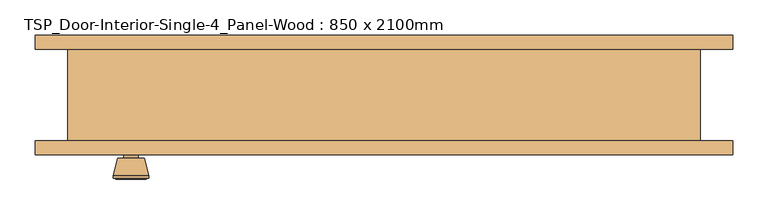
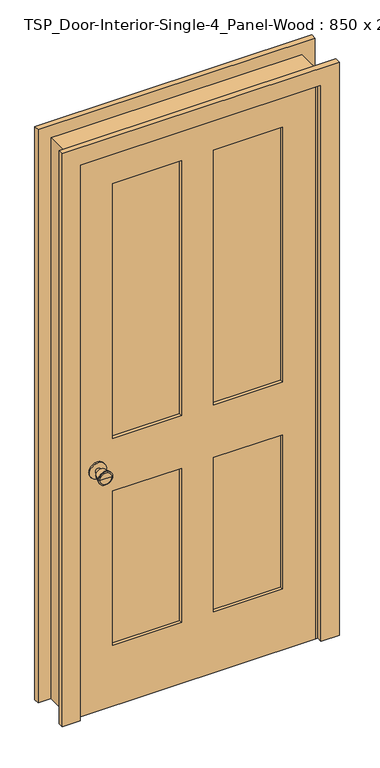
"""IFC4 building model written with IfcOpenShell, lengths in millimetres: door geometry, TSP_Door-Interior-Single-4_Panel-Wood : 850 x 2100mm."""

from ifc_helpers import new_model, si_unit, point, frame, frame_2d, origin, place, context, project, spatial, polyline, circle_curve, trimmed, segment, composite_curve, outline, extrude, faceted_brep, source, transform, mapped, element, save
from ifc_brep_helpers import plane_surface, cylinder_surface, revolved_surface, advanced_brep


def tsp_door_interior_single_4_panel_wood_850_x_2100mm_3b2ec1ce(model_context):
    return source(origin(), model_context, "Body", "SolidModel", [
        advanced_brep(
        [(-360.0, -20.825, 914.4), (-370.0, -20.825, 914.4), (-350.0, -20.825, 914.4), (-339.5241324, 28.175, 914.4), (-380.4758676, 28.175, 914.4), (-360.0, 28.175, 914.4), (-335.0, 26.3471319, 914.4), (-385.0, 26.3471319, 914.4), (-335.0, 22.8834537, 914.4), (-385.0, 22.8834537, 914.4), (-341.363764, -1.825, 914.4), (-378.636236, -1.825, 914.4), (-350.0, -1.825, 914.4), (-370.0, -1.825, 914.4)],
        [
            (0, 1),
            (1, 2, circle_curve(frame((-360.0, -20.825, 914.4), z_axis=(0.0, -1.0, 0.0), x_axis=(-1.0, 0.0, 0.0)), 10.0)),
            (2, 0),
            (2, 1, circle_curve(frame((-360.0, -20.825, 914.4), z_axis=(0.0, -1.0, 0.0), x_axis=(-1.0, 0.0, 0.0)), 10.0)),
            (3, 4, circle_curve(frame((-360.0, 28.175, 914.4), z_axis=(0.0, 1.0, 0.0), x_axis=(-1.0, 0.0, 0.0)), 20.4758676)),
            (4, 5),
            (5, 3),
            (4, 3, circle_curve(frame((-360.0, 28.175, 914.4), z_axis=(0.0, 1.0, 0.0), x_axis=(-1.0, 0.0, 0.0)), 20.4758676)),
            (6, 7, circle_curve(frame((-360.0, 26.3471319, 914.4), z_axis=(0.0, 1.0, 0.0), x_axis=(-1.0, 0.0, 0.0)), 25.0)),
            (7, 4),
            (3, 6),
            (7, 6, circle_curve(frame((-360.0, 26.3471319, 914.4), z_axis=(0.0, 1.0, 0.0), x_axis=(-1.0, 0.0, 0.0)), 25.0)),
            (8, 9, circle_curve(frame((-360.0, 22.8834537, 914.4), z_axis=(0.0, 1.0, 0.0), x_axis=(-1.0, 0.0, 0.0)), 25.0)),
            (9, 7),
            (6, 8),
            (9, 8, circle_curve(frame((-360.0, 22.8834537, 914.4), z_axis=(0.0, 1.0, 0.0), x_axis=(-1.0, 0.0, 0.0)), 25.0)),
            (10, 11, circle_curve(frame((-360.0, -1.825, 914.4), z_axis=(0.0, 1.0, 0.0), x_axis=(-1.0, 0.0, 0.0)), 18.636236)),
            (11, 9),
            (8, 10),
            (11, 10, circle_curve(frame((-360.0, -1.825, 914.4), z_axis=(0.0, 1.0, 0.0), x_axis=(-1.0, 0.0, 0.0)), 18.636236)),
            (12, 13, circle_curve(frame((-360.0, -1.825, 914.4), z_axis=(0.0, 1.0, 0.0), x_axis=(-1.0, 0.0, 0.0)), 10.0)),
            (13, 11),
            (10, 12),
            (13, 12, circle_curve(frame((-360.0, -1.825, 914.4), z_axis=(0.0, 1.0, 0.0), x_axis=(-1.0, 0.0, 0.0)), 10.0)),
            (1, 13),
            (12, 2),
        ],
        [
            plane_surface(frame((-360.0, -20.825, 914.4), z_axis=(0.0, -1.0, 0.0), x_axis=(-1.0, 0.0, 0.0))),
            plane_surface(frame((-360.0, 28.175, 914.4), z_axis=(0.0, 1.0, 0.0), x_axis=(-1.0, 0.0, 0.0))),
            revolved_surface(polyline([(-380.4758676, 28.175, 914.4), (-385.0, 26.3471319, 914.4)]), (-360.0, -20.825, 914.4), (0.0, -1.0, 0.0)),
            cylinder_surface(frame((-360.0, -20.825, 914.4), z_axis=(0.0, -1.0, 0.0), x_axis=(-1.0, 0.0, 0.0)), 25.0),
            revolved_surface(polyline([(-385.0, 22.8834537, 914.4), (-378.636236, -1.825, 914.4)]), (-360.0, -20.825, 914.4), (0.0, -1.0, 0.0)),
            plane_surface(frame((-360.0, -1.825, 914.4), z_axis=(0.0, -1.0, 0.0), x_axis=(-1.0, 0.0, 0.0))),
            cylinder_surface(frame((-360.0, -20.825, 914.4), z_axis=(0.0, -1.0, 0.0), x_axis=(-1.0, 0.0, 0.0)), 10.0),
        ],
        [
            (0, [[1, 2, 3]]),
            (0, [[-3, 4, -1]]),
            (1, [[5, 6, 7]]),
            (1, [[8, -7, -6]]),
            (2, [[9, 10, -5, 11]]),
            (2, [[12, -11, -8, -10]]),
            (3, [[13, 14, -9, 15]]),
            (3, [[16, -15, -12, -14]]),
            (4, [[17, 18, -13, 19]]),
            (4, [[20, -19, -16, -18]]),
            (5, [[21, 22, -17, 23]]),
            (5, [[24, -23, -20, -22]]),
            (6, [[-2, 25, -21, 26]]),
            (6, [[-4, -26, -24, -25]]),
        ],
    ),
        extrude(outline(composite_curve([segment(trimmed(circle_curve(frame_2d((914.4, -360.0)), 30.0), [point((914.4, -390.0))], [point((914.4, -330.0))], False, "CARTESIAN"), True, "CONTINUOUS"), segment(trimmed(circle_curve(frame_2d((914.4, -360.0)), 30.0), [point((914.4, -330.0))], [point((914.4, -390.0))], False, "CARTESIAN"), True, "CONTINUOUS")], self_intersect=False)), frame((0.0, -26.825, 0.0), z_axis=(0.0, 1.0, 0.0), x_axis=(0.0, 0.0, 1.0)), (0.0, 0.0, 1.0), 6.0),
        advanced_brep(
        [(-360.0, -67.825, 914.4), (-350.0, -67.825, 914.4), (-370.0, -67.825, 914.4), (-339.5241324, -116.825, 914.4), (-360.0, -116.825, 914.4), (-380.4758676, -116.825, 914.4), (-335.0, -114.9971319, 914.4), (-385.0, -114.9971319, 914.4), (-335.0, -111.5334537, 914.4), (-385.0, -111.5334537, 914.4), (-341.363764, -86.825, 914.4), (-378.636236, -86.825, 914.4), (-350.0, -86.825, 914.4), (-370.0, -86.825, 914.4)],
        [
            (0, 1),
            (1, 2, circle_curve(frame((-360.0, -67.825, 914.4), z_axis=(0.0, 1.0, 0.0), x_axis=(-1.0, 0.0, 0.0)), 10.0)),
            (2, 0),
            (2, 1, circle_curve(frame((-360.0, -67.825, 914.4), z_axis=(0.0, 1.0, 0.0), x_axis=(-1.0, 0.0, 0.0)), 10.0)),
            (3, 4),
            (4, 5),
            (5, 3, circle_curve(frame((-360.0, -116.825, 914.4), z_axis=(0.0, -1.0, 0.0), x_axis=(-1.0, 0.0, 0.0)), 20.4758676)),
            (3, 5, circle_curve(frame((-360.0, -116.825, 914.4), z_axis=(0.0, -1.0, 0.0), x_axis=(-1.0, 0.0, 0.0)), 20.4758676)),
            (6, 3),
            (5, 7),
            (7, 6, circle_curve(frame((-360.0, -114.9971319, 914.4), z_axis=(0.0, -1.0, 0.0), x_axis=(-1.0, 0.0, 0.0)), 25.0)),
            (6, 7, circle_curve(frame((-360.0, -114.9971319, 914.4), z_axis=(0.0, -1.0, 0.0), x_axis=(-1.0, 0.0, 0.0)), 25.0)),
            (8, 6),
            (7, 9),
            (9, 8, circle_curve(frame((-360.0, -111.5334537, 914.4), z_axis=(0.0, -1.0, 0.0), x_axis=(-1.0, 0.0, 0.0)), 25.0)),
            (8, 9, circle_curve(frame((-360.0, -111.5334537, 914.4), z_axis=(0.0, -1.0, 0.0), x_axis=(-1.0, 0.0, 0.0)), 25.0)),
            (10, 8),
            (9, 11),
            (11, 10, circle_curve(frame((-360.0, -86.825, 914.4), z_axis=(0.0, -1.0, 0.0), x_axis=(-1.0, 0.0, 0.0)), 18.636236)),
            (10, 11, circle_curve(frame((-360.0, -86.825, 914.4), z_axis=(0.0, -1.0, 0.0), x_axis=(-1.0, 0.0, 0.0)), 18.636236)),
            (12, 10),
            (11, 13),
            (13, 12, circle_curve(frame((-360.0, -86.825, 914.4), z_axis=(0.0, -1.0, 0.0), x_axis=(-1.0, 0.0, 0.0)), 10.0)),
            (12, 13, circle_curve(frame((-360.0, -86.825, 914.4), z_axis=(0.0, -1.0, 0.0), x_axis=(-1.0, 0.0, 0.0)), 10.0)),
            (1, 12),
            (13, 2),
        ],
        [
            plane_surface(frame((-360.0, -67.825, 914.4), z_axis=(0.0, 1.0, 0.0), x_axis=(-1.0, 0.0, 0.0))),
            plane_surface(frame((-360.0, -116.825, 914.4), z_axis=(0.0, -1.0, 0.0), x_axis=(-1.0, 0.0, 0.0))),
            revolved_surface(polyline([(-380.4758676, -116.825, 914.4), (-385.0, -114.9971319, 914.4)]), (-360.0, -67.825, 914.4), (0.0, 1.0, 0.0)),
            cylinder_surface(frame((-360.0, -67.825, 914.4), z_axis=(0.0, 1.0, 0.0), x_axis=(-1.0, 0.0, 0.0)), 25.0),
            revolved_surface(polyline([(-385.0, -111.5334537, 914.4), (-378.636236, -86.825, 914.4)]), (-360.0, -67.825, 914.4), (0.0, 1.0, 0.0)),
            plane_surface(frame((-360.0, -86.825, 914.4), z_axis=(0.0, 1.0, 0.0), x_axis=(-1.0, 0.0, 0.0))),
            cylinder_surface(frame((-360.0, -67.825, 914.4), z_axis=(0.0, 1.0, 0.0), x_axis=(-1.0, 0.0, 0.0)), 10.0),
        ],
        [
            (0, [[1, 2, 3]]),
            (0, [[-3, 4, -1]]),
            (1, [[5, 6, 7]]),
            (1, [[-6, -5, 8]]),
            (2, [[9, -7, 10, 11]]),
            (2, [[-10, -8, -9, 12]]),
            (3, [[13, -11, 14, 15]]),
            (3, [[-14, -12, -13, 16]]),
            (4, [[17, -15, 18, 19]]),
            (4, [[-18, -16, -17, 20]]),
            (5, [[21, -19, 22, 23]]),
            (5, [[-22, -20, -21, 24]]),
            (6, [[25, -23, 26, -2]]),
            (6, [[-26, -24, -25, -4]]),
        ],
    ),
        extrude(outline(composite_curve([segment(trimmed(circle_curve(frame_2d((914.4, -360.0)), 30.0), [point((914.4, -390.0))], [point((914.4, -330.0))], False, "CARTESIAN"), True, "CONTINUOUS"), segment(trimmed(circle_curve(frame_2d((914.4, -360.0)), 30.0), [point((914.4, -330.0))], [point((914.4, -390.0))], False, "CARTESIAN"), True, "CONTINUOUS")], self_intersect=False)), frame((0.0, -67.825, 0.0), z_axis=(0.0, 1.0, 0.0), x_axis=(0.0, 0.0, 1.0)), (0.0, 0.0, 1.0), 6.0),
        faceted_brep([(450.0, -61.825, 0.0), (425.0, -61.825, 0.0), (425.0, -26.825, 0.0), (412.3, -26.825, 0.0), (412.3, 8.1, 0.0), (425.0, 8.1, 0.0), (425.0, 68.175, 0.0), (450.0, 68.175, 0.0), (450.0, 68.175, 2125.0), (450.0, -61.825, 2125.0), (425.0, 68.175, 2100.0), (-425.0, 68.175, 2100.0), (-425.0, 68.175, 0.0), (-450.0, 68.175, 0.0), (-450.0, 68.175, 2125.0), (425.0, 8.1, 2100.0), (412.3, 8.1, 2087.3), (-412.3, 8.1, 2087.3), (-412.3, 8.1, 0.0), (-425.0, 8.1, 0.0), (-425.0, 8.1, 2100.0), (412.3, -26.825, 2087.3), (425.0, -26.825, 2100.0), (-425.0, -26.825, 2100.0), (-425.0, -26.825, 0.0), (-412.3, -26.825, 0.0), (-412.3, -26.825, 2087.3), (425.0, -61.825, 2100.0), (-450.0, -61.825, 2125.0), (-450.0, -61.825, 0.0), (-425.0, -61.825, 0.0), (-425.0, -61.825, 2100.0)], [[[0, 1, 2, 3, 4, 5, 6, 7]], [[7, 8, 9, 0]], [[6, 10, 11, 12, 13, 14, 8, 7]], [[5, 15, 10, 6]], [[4, 16, 17, 18, 19, 20, 15, 5]], [[3, 21, 16, 4]], [[2, 22, 23, 24, 25, 26, 21, 3]], [[1, 27, 22, 2]], [[0, 9, 28, 29, 30, 31, 27, 1]], [[8, 14, 28, 9]], [[15, 20, 11, 10]], [[21, 26, 17, 16]], [[27, 31, 23, 22]], [[29, 13, 12, 19, 18, 25, 24, 30]], [[14, 13, 29, 28]], [[20, 19, 12, 11]], [[26, 25, 18, 17]], [[31, 30, 24, 23]]]),
        extrude(outline(polyline([(2100.0, -425.0), (0.0, -425.0), (0.0, 425.0), (2100.0, 425.0), (2100.0, -425.0)]), holes=[polyline([(1980.0, 57.5), (1980.0, 305.0), (1014.4, 305.0), (1014.4, 57.5), (1980.0, 57.5)]), polyline([(1014.4, -57.5), (1014.4, -305.0), (1980.0, -305.0), (1980.0, -57.5), (1014.4, -57.5)]), polyline([(814.4, 57.5), (814.4, 305.0), (230.0, 305.0), (230.0, 57.5), (814.4, 57.5)]), polyline([(230.0, -57.5), (230.0, -305.0), (814.4, -305.0), (814.4, -57.5), (230.0, -57.5)])]), frame((0.0, -61.825, 0.0), z_axis=(0.0, 1.0, 0.0), x_axis=(0.0, 0.0, 1.0)), (0.0, 0.0, 1.0), 35.0),
        extrude(outline(polyline([(305.0, -38.4916667), (305.0, -50.1583333), (57.5, -50.1583333), (57.5, -38.4916667), (305.0, -38.4916667)])), frame((0.0, 0.0, 1014.4), z_axis=(0.0, 0.0, 1.0), x_axis=(1.0, 0.0, 0.0)), (0.0, 0.0, 1.0), 965.6),
        extrude(outline(polyline([(-57.5, -38.4916667), (-57.5, -50.1583333), (-305.0, -50.1583333), (-305.0, -38.4916667), (-57.5, -38.4916667)])), frame((0.0, 0.0, 1014.4), z_axis=(0.0, 0.0, 1.0), x_axis=(1.0, 0.0, 0.0)), (0.0, 0.0, 1.0), 965.6),
        extrude(outline(polyline([(305.0, -38.4916667), (305.0, -50.1583333), (57.5, -50.1583333), (57.5, -38.4916667), (305.0, -38.4916667)])), frame((0.0, 0.0, 230.0), z_axis=(0.0, 0.0, 1.0), x_axis=(1.0, 0.0, 0.0)), (0.0, 0.0, 1.0), 584.4),
        extrude(outline(polyline([(-57.5, -38.4916667), (-57.5, -50.1583333), (-305.0, -50.1583333), (-305.0, -38.4916667), (-57.5, -38.4916667)])), frame((0.0, 0.0, 230.0), z_axis=(0.0, 0.0, 1.0), x_axis=(1.0, 0.0, 0.0)), (0.0, 0.0, 1.0), 584.4),
        extrude(outline(polyline([(0.0, 496.35), (2171.35, 496.35), (2171.35, -496.35), (0.0, -496.35), (0.0, -431.35), (2106.35, -431.35), (2106.35, 431.35), (0.0, 431.35), (0.0, 496.35)])), frame((0.0, -81.825, 0.0), z_axis=(0.0, 1.0, 0.0), x_axis=(0.0, 0.0, 1.0)), (0.0, 0.0, 1.0), 20.0),
        extrude(outline(polyline([(0.0, 496.35), (2171.35, 496.35), (2171.35, -496.35), (0.0, -496.35), (0.0, -431.35), (2106.35, -431.35), (2106.35, 431.35), (0.0, 431.35), (0.0, 496.35)])), frame((0.0, 68.175, 0.0), z_axis=(0.0, 1.0, 0.0), x_axis=(0.0, 0.0, 1.0)), (0.0, 0.0, 1.0), 20.0),
    ])


if __name__ == "__main__":
    model = new_model("IFC4")
    model_context = context("Model", 3, world=origin())
    ifc_project = project(units=[si_unit("LENGTHUNIT", "METRE", prefix="MILLI")], contexts=[model_context])
    site = spatial("IfcSite", under=ifc_project)
    building = spatial("IfcBuilding", under=site)
    placement = place(None, origin())
    tsp_door_interior_single_4_panel_wood_850_x_2100mm_shape = tsp_door_interior_single_4_panel_wood_850_x_2100mm_3b2ec1ce(model_context)
    element("IfcDoor", 1, ObjectType="TSP_Door-Interior-Single-4_Panel-Wood : 850 x 2100mm", at=placement, inside=building, context=model_context, shape_type="MappedRepresentation", body=[
        mapped(tsp_door_interior_single_4_panel_wood_850_x_2100mm_shape, transform((0.0, 0.0, 0.0), x_axis=(1.0, 0.0, 0.0), y_axis=(0.0, 1.0, 0.0), z_axis=(0.0, 0.0, 1.0))),
    ])
    save(model, "model.ifc")

# Revit data of these elements
# Type "TSP_Door-Interior-Single-4_Panel-Wood : 850 x 2100mm"
#   Model = "TSP_DOOR02W"
#   Type Mark = "243"
#   Assembly Code = "C1020300"
#   Analytic Construction = "Wooden"
#   Top Rail = 120 mm
#   Thickness = 35 mm
#   Thermal Resistance (R) = 0.455703 (m²·K)/W
#   Swing Angle [instance default] = 90.00°
#   Stiles = 120 mm
#   Rough Width = 900 mm
#   Rough Height = 2125 mm
#   Mullion = 115 mm
#   Lock Rail = 200 mm
#   Height = 2100 mm
#   Width = 850 mm
#   Heat Transfer Coefficient (U) = 2.19465 W/(m²·K)
#   Bottom Rail = 230 mm
#   Define Thermal Properties by = 1
#   Trim Material = Cherry
#   Panel Material = Cherry
#   Frame Material = Cherry
#   Door Handle Material = Aluminum
#   Visual Light Transmittance = 0
#   Solar Heat Gain Coefficient = 0
#   Wall Closure = (empty or 0)
#   Function = (empty or 0)
# Element 1 (IfcDoor, "TSP_Door-Interior-Single-4_Panel-Wood : 850 x 2100mm")
#   Materials on its faces: "Cherry", "Aluminum"
# Materials
#   "Cherry": class "Wood", colour RGB 226 177 128, transparency 0, Description = "Prunus Serotina", Cost = 0
#   "Aluminum": class "Metal", colour RGB 247 247 247, transparency 0, Description = "Aluminum 6061", Cost = 0
